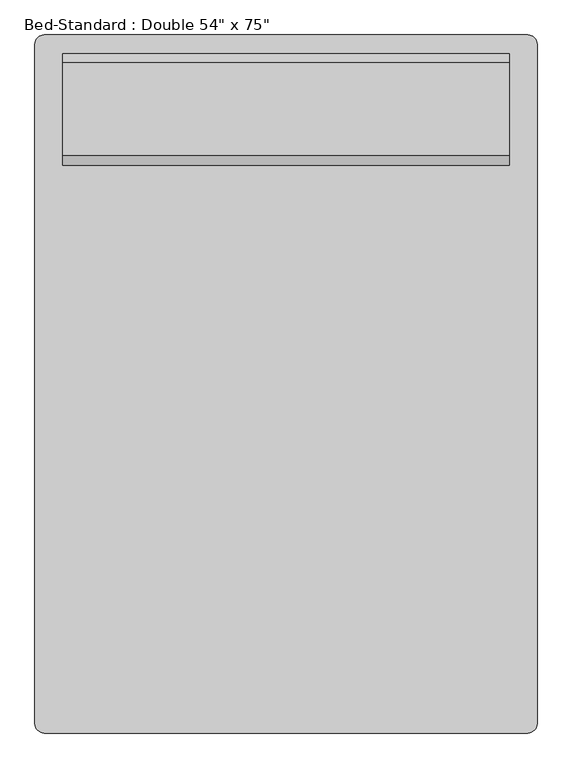
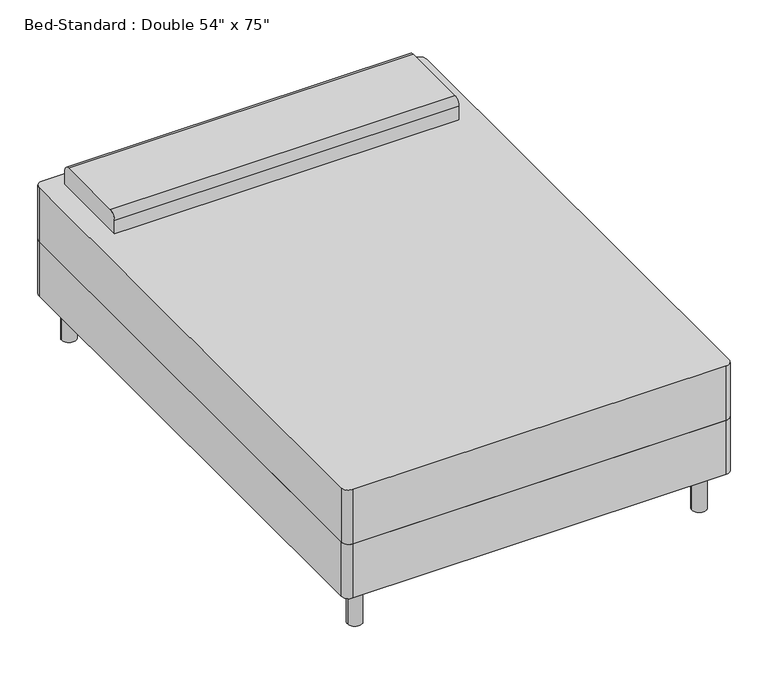
"""IFC4 building model written with IfcOpenShell, lengths in millimetres: furniture geometry."""

import ifcopenshell
import ifcopenshell.guid

model = None  # the IFC model being written
_history = None  # IfcOwnerHistory: only IFC2X3 demands one
_inside = {}  # id of a spatial element -> (the spatial element, [elements in it])
_under = {}  # id of a project, library or spatial element -> (it, [spatial elements below it])
_declared = {}  # id of a project -> (the project, [libraries it declares])
_typed = {}  # id of a type object -> (the type object, [elements of that type])
_made_of = {}  # id of a material, layer set ... -> (it, [elements and type objects made of it])


def new_model(schema):
    """Start an empty IFC model of exactly this schema.

    Asked for "IFC4X3", IfcOpenShell would pick the latest addendum, in which some entities
    have other attributes; the version numbers below select the first issue.
    IFC2X3 requires an IfcOwnerHistory on every rooted entity: one is made here for all.
    """
    global model, _history
    if schema == "IFC4X3":
        model = ifcopenshell.file(schema_version=(4, 3, 0, 0))
    else:
        model = ifcopenshell.file(schema=schema)
    _inside.clear()
    _under.clear()
    _declared.clear()
    _typed.clear()
    _made_of.clear()
    _history = None
    if model.schema == "IFC2X3":
        org = make("IfcOrganization", Name="unknown")
        user = make(
            "IfcPersonAndOrganization",
            ThePerson=make("IfcPerson", FamilyName="unknown"),
            TheOrganization=org,
        )
        app = make(
            "IfcApplication",
            ApplicationDeveloper=org,
            Version="unknown",
            ApplicationFullName="unknown",
            ApplicationIdentifier="unknown",
        )
        _history = make(
            "IfcOwnerHistory",
            OwningUser=user,
            OwningApplication=app,
            ChangeAction="ADDED",
            CreationDate=0,
        )
    return model


def make(cls, **values):
    """One entity of the class cls with the attributes given. An attribute that is None is left unset."""
    return model.create_entity(
        cls, **{name: value for name, value in values.items() if value is not None}
    )


def rooted(cls, **values):
    """An entity with a GlobalId (a new one), such as an element, a storey or a relation."""
    return make(cls, GlobalId=ifcopenshell.guid.new(), OwnerHistory=_history, **values)


def si_unit(unit_type, name, prefix=None):
    """IfcSIUnit, for example si_unit("LENGTHUNIT", "METRE", prefix="MILLI")."""
    return make("IfcSIUnit", UnitType=unit_type, Prefix=prefix, Name=name)


def assignment(units):
    """IfcUnitAssignment: the units of a project."""
    return None if units is None else make("IfcUnitAssignment", Units=units)


def point(xyz):
    """IfcCartesianPoint."""
    return None if xyz is None else make("IfcCartesianPoint", Coordinates=xyz)


def direction(xyz):
    """IfcDirection."""
    return None if xyz is None else make("IfcDirection", DirectionRatios=xyz)


def frame(location, z_axis=None, x_axis=None):
    """IfcAxis2Placement3D, a coordinate frame: its origin and axes. An axis left out is left unset."""
    return make(
        "IfcAxis2Placement3D",
        Location=point(location),
        Axis=direction(z_axis),
        RefDirection=direction(x_axis),
    )


def frame_2d(location, x_axis=None):
    """IfcAxis2Placement2D, a coordinate frame in the plane: its origin and x axis."""
    return make(
        "IfcAxis2Placement2D", Location=point(location), RefDirection=direction(x_axis)
    )


def origin():
    """The frame at (0, 0, 0) with its axes left unset."""
    return frame((0.0, 0.0, 0.0))


def origin_with_axes():
    """The frame at (0, 0, 0) with the z axis (0, 0, 1) and the x axis (1, 0, 0) written out."""
    return frame((0.0, 0.0, 0.0), z_axis=(0.0, 0.0, 1.0), x_axis=(1.0, 0.0, 0.0))


def place(relative_to, where):
    """IfcLocalPlacement: puts the frame where relative to a parent placement (None: the world)."""
    return make(
        "IfcLocalPlacement", PlacementRelTo=relative_to, RelativePlacement=where
    )


def context(
    kind, dimensions, precision=None, world=None, true_north=None, identifier=None
):
    """IfcGeometricRepresentationContext, for example the 3D "Model" context."""
    return make(
        "IfcGeometricRepresentationContext",
        ContextIdentifier=identifier,
        ContextType=kind,
        CoordinateSpaceDimension=dimensions,
        Precision=precision,
        WorldCoordinateSystem=world,
        TrueNorth=true_north,
    )


def project(units=None, contexts=None):
    """IfcProject with its units and contexts."""
    return rooted(
        "IfcProject",
        Name="project",
        RepresentationContexts=contexts,
        UnitsInContext=assignment(units),
    )


def spatial(cls, under=None, at=None, **own):
    """A site, building, storey or space (cls), placed at a placement, below another one or the project."""
    s = rooted(cls, ObjectPlacement=at, **own)
    if under is not None:
        _under.setdefault(under.id(), (under, []))[1].append(s)
    return s


def polyline(points):
    """IfcPolyline through the points."""
    return make("IfcPolyline", Points=[point(p) for p in points])


def circle_curve(where, radius):
    """IfcCircle in the frame where."""
    return make("IfcCircle", Position=where, Radius=radius)


def trimmed(basis, trim1, trim2, sense, master):
    """IfcTrimmedCurve: the piece of a basis curve between two trims."""
    return make(
        "IfcTrimmedCurve",
        BasisCurve=basis,
        Trim1=trim1,
        Trim2=trim2,
        SenseAgreement=sense,
        MasterRepresentation=master,
    )


def segment(curve, same_sense, transition):
    """IfcCompositeCurveSegment."""
    return make(
        "IfcCompositeCurveSegment",
        Transition=transition,
        SameSense=same_sense,
        ParentCurve=curve,
    )


def composite_curve(segments, self_intersect=None):
    """IfcCompositeCurve: segments joined end to end."""
    return make("IfcCompositeCurve", Segments=segments, SelfIntersect=self_intersect)


def outline(outer, holes=None, kind="AREA"):
    """IfcArbitraryClosedProfileDef: a profile drawn as a closed curve; with holes, ...WithVoids."""
    if holes is None:
        return make("IfcArbitraryClosedProfileDef", ProfileType=kind, OuterCurve=outer)
    return make(
        "IfcArbitraryProfileDefWithVoids",
        ProfileType=kind,
        OuterCurve=outer,
        InnerCurves=holes,
    )


def extrude(swept, where, along, depth):
    """IfcExtrudedAreaSolid: the profile swept, set in the frame where, extruded along a direction by depth."""
    return make(
        "IfcExtrudedAreaSolid",
        SweptArea=swept,
        Position=where,
        ExtrudedDirection=direction(along),
        Depth=depth,
    )


def shape(context_of_items, identifier, shape_type, items):
    """IfcShapeRepresentation: the items that make up one representation, for example the "Body"."""
    return make(
        "IfcShapeRepresentation",
        ContextOfItems=context_of_items,
        RepresentationIdentifier=identifier,
        RepresentationType=shape_type,
        Items=items,
    )


def source(mapping_origin, context_of_items, identifier, shape_type, items):
    """IfcRepresentationMap: a shape defined once, which mapped items show again and again."""
    return make(
        "IfcRepresentationMap",
        MappingOrigin=mapping_origin,
        MappedRepresentation=shape(context_of_items, identifier, shape_type, items),
    )


def transform(
    local_origin,
    x_axis=None,
    y_axis=None,
    z_axis=None,
    scale=None,
    scale2=None,
    scale3=None,
    uniform=True,
):
    """IfcCartesianTransformationOperator3D, or its non-uniform kind. x_axis, y_axis, z_axis: its Axis1, 2, 3."""
    if uniform:
        return make(
            "IfcCartesianTransformationOperator3D",
            Axis1=direction(x_axis),
            Axis2=direction(y_axis),
            LocalOrigin=point(local_origin),
            Scale=scale,
            Axis3=direction(z_axis),
        )
    return make(
        "IfcCartesianTransformationOperator3DnonUniform",
        Axis1=direction(x_axis),
        Axis2=direction(y_axis),
        LocalOrigin=point(local_origin),
        Scale=scale,
        Axis3=direction(z_axis),
        Scale2=scale2,
        Scale3=scale3,
    )


def mapped(mapping_source, mapping_target):
    """IfcMappedItem: shows the shape of a source again, moved by a transform."""
    return make(
        "IfcMappedItem", MappingSource=mapping_source, MappingTarget=mapping_target
    )


def made_of(thing, what):
    """Note that an element or type object is made of a material, layer set ...; save() writes the relation."""
    if what is not None:
        _made_of.setdefault(what.id(), (what, []))[1].append(thing)
    return thing


def element(
    cls,
    number,
    at=None,
    inside=None,
    cuts=None,
    type_object=None,
    material=None,
    context=None,
    identifier="Body",
    shape_type=None,
    held_by="IfcProductDefinitionShape",
    body=None,
    shapes=None,
    **own,
):
    """One element of the class cls, such as IfcWall. Its Tag is "e" and its number.

    at: its placement. inside: the storey or other place that contains it. cuts: it is an
    opening in that element (IfcRelVoidsElement). A single representation is given by context,
    identifier, shape_type and body (its items); several are given by shapes. held_by: the class
    of the entity that holds the representations. save() writes the other relations.
    """
    e = rooted(cls, Tag="e%d" % number, ObjectPlacement=at, **own)
    if body is not None:
        shapes = [shape(context, identifier, shape_type, body)]
    if shapes is not None:
        e.Representation = make(held_by, Representations=shapes)
    if inside is not None:
        _inside.setdefault(inside.id(), (inside, []))[1].append(e)
    if cuts is not None:
        rooted(
            "IfcRelVoidsElement", RelatingBuildingElement=cuts, RelatedOpeningElement=e
        )
    if type_object is not None:
        _typed.setdefault(type_object.id(), (type_object, []))[1].append(e)
    return made_of(e, material)


def aggregate(whole, parts):
    """IfcRelAggregates: a whole, such as a stair, and the parts it consists of."""
    return rooted("IfcRelAggregates", RelatingObject=whole, RelatedObjects=parts)


def save(model, path):
    """Write the relations noted so far, then the file.

    IfcRelAggregates (storeys below a building ...), IfcRelContainedInSpatialStructure (elements
    in a storey), IfcRelDefinesByType, IfcRelAssociatesMaterial and IfcRelDeclares: one each for
    every whole, place, type object, material and project.
    """
    for whole, parts in _under.values():
        aggregate(whole, parts)
    for where, things in _inside.values():
        rooted(
            "IfcRelContainedInSpatialStructure",
            RelatedElements=things,
            RelatingStructure=where,
        )
    for kind, things in _typed.values():
        rooted("IfcRelDefinesByType", RelatedObjects=things, RelatingType=kind)
    for what, things in _made_of.values():
        rooted("IfcRelAssociatesMaterial", RelatedObjects=things, RelatingMaterial=what)
    for by, libraries in _declared.values():
        rooted("IfcRelDeclares", RelatingContext=by, RelatedDefinitions=libraries)
    model.write(path)


def furniture_52ef1662(model_context):
    return source(origin(), model_context, "Body", "SweptSolid", [
        extrude(outline(composite_curve([segment(polyline([(-388.9114754, 906.904918), (931.8885246, 906.904918)]), True, "CONTINUOUS"), segment(trimmed(circle_curve(frame_2d((931.8885246, 881.504918)), 25.4), [point((931.8885246, 906.904918))], [point((957.2885246, 881.504918))], False, "CARTESIAN"), True, "CONTINUOUS"), segment(polyline([(957.2885246, 881.504918), (957.2885246, -972.695082)]), True, "CONTINUOUS"), segment(trimmed(circle_curve(frame_2d((931.8885246, -972.695082)), 25.4), [point((957.2885246, -972.695082))], [point((931.8885246, -998.095082))], False, "CARTESIAN"), True, "CONTINUOUS"), segment(polyline([(931.8885246, -998.095082), (-388.9114754, -998.095082)]), True, "CONTINUOUS"), segment(trimmed(circle_curve(frame_2d((-388.9114754, -972.695082)), 25.4), [point((-388.9114754, -998.095082))], [point((-414.3114754, -972.695082))], False, "CARTESIAN"), True, "CONTINUOUS"), segment(polyline([(-414.3114754, -972.695082), (-414.3114754, 881.504918)]), True, "CONTINUOUS"), segment(trimmed(circle_curve(frame_2d((-388.9114754, 881.504918)), 25.4), [point((-414.3114754, 881.504918))], [point((-388.9114754, 906.904918))], False, "CARTESIAN"), True, "CONTINUOUS")], self_intersect=False)), frame((0.0, 0.0, 355.6), z_axis=(0.0, 0.0, 1.0), x_axis=(1.0, 0.0, 0.0)), (0.0, 0.0, 1.0), 203.2),
        extrude(outline(composite_curve([segment(trimmed(circle_curve(frame_2d((-338.1114754, 830.704918)), 25.4), [point((-363.5114754, 830.704918))], [point((-312.7114754, 830.704918))], False, "CARTESIAN"), True, "CONTINUOUS"), segment(trimmed(circle_curve(frame_2d((-338.1114754, 830.704918)), 25.4), [point((-312.7114754, 830.704918))], [point((-363.5114754, 830.704918))], False, "CARTESIAN"), True, "CONTINUOUS")], self_intersect=False)), origin_with_axes(), (0.0, 0.0, 1.0), 152.4),
        extrude(outline(composite_curve([segment(trimmed(circle_curve(frame_2d((881.0885246, 830.704918)), 25.4), [point((855.6885246, 830.704918))], [point((906.4885246, 830.704918))], False, "CARTESIAN"), True, "CONTINUOUS"), segment(trimmed(circle_curve(frame_2d((881.0885246, 830.704918)), 25.4), [point((906.4885246, 830.704918))], [point((855.6885246, 830.704918))], False, "CARTESIAN"), True, "CONTINUOUS")], self_intersect=False)), origin_with_axes(), (0.0, 0.0, 1.0), 152.4),
        extrude(outline(composite_curve([segment(trimmed(circle_curve(frame_2d((881.0885246, -921.895082)), 25.4), [point((855.6885246, -921.895082))], [point((906.4885246, -921.895082))], False, "CARTESIAN"), True, "CONTINUOUS"), segment(trimmed(circle_curve(frame_2d((881.0885246, -921.895082)), 25.4), [point((906.4885246, -921.895082))], [point((855.6885246, -921.895082))], False, "CARTESIAN"), True, "CONTINUOUS")], self_intersect=False)), origin_with_axes(), (0.0, 0.0, 1.0), 152.4),
        extrude(outline(composite_curve([segment(trimmed(circle_curve(frame_2d((-338.1114754, -921.895082)), 25.4), [point((-363.5114754, -921.895082))], [point((-312.7114754, -921.895082))], False, "CARTESIAN"), True, "CONTINUOUS"), segment(trimmed(circle_curve(frame_2d((-338.1114754, -921.895082)), 25.4), [point((-312.7114754, -921.895082))], [point((-363.5114754, -921.895082))], False, "CARTESIAN"), True, "CONTINUOUS")], self_intersect=False)), origin_with_axes(), (0.0, 0.0, 1.0), 152.4),
        extrude(outline(composite_curve([segment(polyline([(551.304918, 558.8), (551.304918, 609.6)]), True, "CONTINUOUS"), segment(trimmed(circle_curve(frame_2d((576.704918, 609.6)), 25.4), [point((551.304918, 609.6))], [point((576.704918, 635.0))], False, "CARTESIAN"), True, "CONTINUOUS"), segment(polyline([(576.704918, 635.0), (830.704918, 635.0)]), True, "CONTINUOUS"), segment(trimmed(circle_curve(frame_2d((830.704918, 609.6)), 25.4), [point((830.704918, 635.0))], [point((856.104918, 609.6))], False, "CARTESIAN"), True, "CONTINUOUS"), segment(polyline([(856.104918, 609.6), (856.104918, 558.8), (551.304918, 558.8)]), True, "CONTINUOUS")], self_intersect=False)), frame((-338.1114754, 0.0, 0.0), z_axis=(1.0, 0.0, 0.0), x_axis=(0.0, 1.0, 0.0)), (0.0, 0.0, 1.0), 1219.2),
        extrude(outline(composite_curve([segment(polyline([(-414.3114754, -972.695082), (-414.3114754, 881.504918)]), True, "CONTINUOUS"), segment(trimmed(circle_curve(frame_2d((-388.9114754, 881.504918)), 25.4), [point((-414.3114754, 881.504918))], [point((-388.9114754, 906.904918))], False, "CARTESIAN"), True, "CONTINUOUS"), segment(polyline([(-388.9114754, 906.904918), (931.8885246, 906.904918)]), True, "CONTINUOUS"), segment(trimmed(circle_curve(frame_2d((931.8885246, 881.504918)), 25.4), [point((931.8885246, 906.904918))], [point((957.2885246, 881.504918))], False, "CARTESIAN"), True, "CONTINUOUS"), segment(polyline([(957.2885246, 881.504918), (957.2885246, -972.695082)]), True, "CONTINUOUS"), segment(trimmed(circle_curve(frame_2d((931.8885246, -972.695082)), 25.4), [point((957.2885246, -972.695082))], [point((931.8885246, -998.095082))], False, "CARTESIAN"), True, "CONTINUOUS"), segment(polyline([(931.8885246, -998.095082), (-388.9114754, -998.095082)]), True, "CONTINUOUS"), segment(trimmed(circle_curve(frame_2d((-388.9114754, -972.695082)), 25.4), [point((-388.9114754, -998.095082))], [point((-414.3114754, -972.695082))], False, "CARTESIAN"), True, "CONTINUOUS")], self_intersect=False)), frame((0.0, 0.0, 152.4), z_axis=(0.0, 0.0, 1.0), x_axis=(1.0, 0.0, 0.0)), (0.0, 0.0, 1.0), 203.2),
    ])


if __name__ == "__main__":
    model = new_model("IFC4")
    model_context = context("Model", 3, world=origin())
    ifc_project = project(units=[si_unit("LENGTHUNIT", "METRE", prefix="MILLI")], contexts=[model_context])
    site = spatial("IfcSite", under=ifc_project)
    building = spatial("IfcBuilding", under=site)
    placement = place(None, origin())
    furniture_shape = furniture_52ef1662(model_context)
    element("IfcFurniture", 1, ObjectType="Bed-Standard : Double 54\" x 75\"", at=placement, inside=building, context=model_context, shape_type="MappedRepresentation", body=[
        mapped(furniture_shape, transform((0.0, 0.0, 0.0), x_axis=(1.0, 0.0, 0.0), y_axis=(0.0, 1.0, 0.0), z_axis=(0.0, 0.0, 1.0))),
    ])
    save(model, "model.ifc")

# Revit data of these elements
# Project information
#   Project Issue Date = "Issue Date"
#   Project Status = "Project Status"
#   Client Name = "Owner"
#   Project Address = "Enter address here"
#   Project Name = "Project Name"
#   Project Number = "Project Number"
# Type "Bed-Standard : Double 54\" x 75\""
#   Assembly Code = "E2020200"
#   Length = 6' - 3"
#   Width = 4' - 6"
#   Leg Material = Steel, Chrome Plated
#   Mattress Material = Linen, White
#   Default Elevation = 0
# Element 1 (IfcFurniture, "Bed-Standard : Double 54\" x 75\"")
#   Materials on its faces: "Linen, White", "Steel, Chrome Plated"
# Materials
#   "Steel, Chrome Plated": class "Metal", colour RGB 17 17 17, transparency 0, Description = "Chromiuim plated steel", Cost = 0
#   "Linen, White": class "Textile", colour RGB 247 247 239, transparency 0, Description = "Linen, white", Cost = 0
